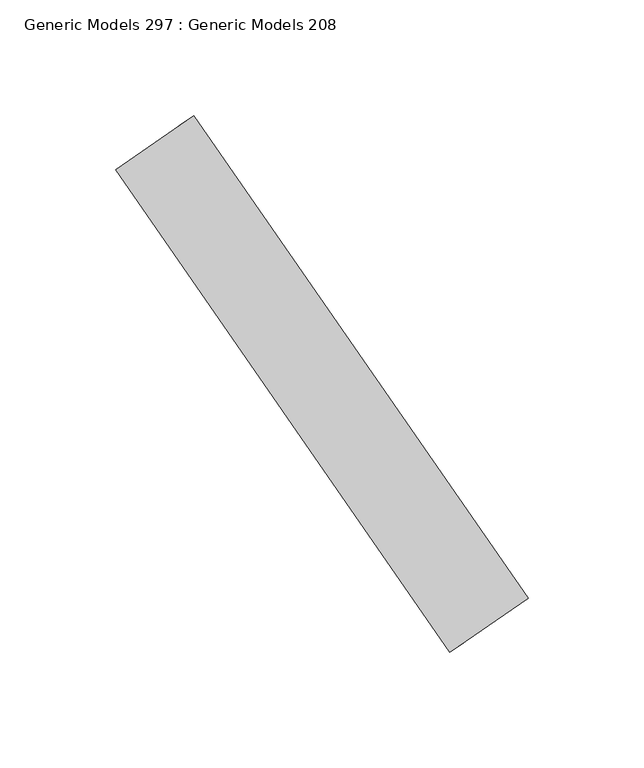
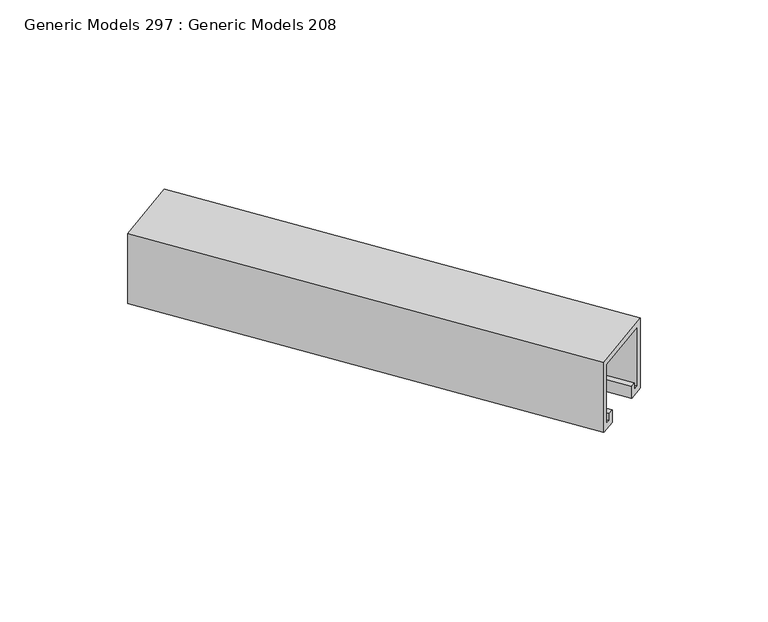
"""IFC4 building model written with IfcOpenShell, lengths in millimetres: proxy geometry, Generic Models 297 : Generic Models 208."""

from ifc_helpers import new_model, si_unit, frame, origin, place, context, project, spatial, polyline, outline, extrude, source, transform, mapped, element, save


def generic_models_297_generic_models_208_0078fd4a(model_context):
    return source(origin(), model_context, "Body", "SweptSolid", [
        extrude(outline(polyline([(-3.175, 0.0), (-3.175, 34.925), (-38.1, 34.925), (-38.1, 31.75), (-34.13125, 31.75), (-34.13125, 28.5750001), (-41.275, 28.5750001), (-41.275, 38.1), (0.0, 38.1), (0.0, -3.175), (-41.275, -3.175), (-41.275, 6.35), (-34.13125, 6.35), (-34.13125, 3.175), (-38.1, 3.175), (-38.1, 0.0), (-3.175, 0.0)])), frame((-2463.8722582, -22814.1902031, 1035.05), z_axis=(-0.5693796736417774, 0.8220746847115432, 0.0), x_axis=(0.0, 0.0, 1.0)), (0.0, 0.0, 1.0), 254.0),
    ])


if __name__ == "__main__":
    model = new_model("IFC4")
    model_context = context("Model", 3, world=origin())
    ifc_project = project(units=[si_unit("LENGTHUNIT", "METRE", prefix="MILLI")], contexts=[model_context])
    site = spatial("IfcSite", under=ifc_project)
    building = spatial("IfcBuilding", under=site)
    placement = place(None, origin())
    generic_models_297_generic_models_208_shape = generic_models_297_generic_models_208_0078fd4a(model_context)
    element("IfcBuildingElementProxy", 1, Name="Generic Models 297 : Generic Models 208", ObjectType="Generic Models 297 : Generic Models 208", at=placement, inside=building, context=model_context, shape_type="MappedRepresentation", body=[
        mapped(generic_models_297_generic_models_208_shape, transform((0.0, 0.0, 0.0), x_axis=(1.0, 0.0, 0.0), y_axis=(0.0, 1.0, 0.0), z_axis=(0.0, 0.0, 1.0))),
    ])
    save(model, "model.ifc")

# Revit data of these elements
# Project information
#   Project Issue Date = "03.10.2017"
#   Project Status = "Project Status"
#   Client Name = "Owner"
#   Project Address = "5964 Executive Dr, Fitchburg, WI 53719"
#   Project Name = "Infinite Athlete"
#   Project Number = "Project Number"
# Element 1 (IfcBuildingElementProxy, "Generic Models 297 : Generic Models 208")
#   Materials on its faces: "UNISTRUT P1000, 1 5/8\" X 1 5/8\", CHANNEL OR ALUM. CHANNEL"
# Materials
#   "UNISTRUT P1000, 1 5/8\" X 1 5/8\", CHANNEL OR ALUM. CHANNEL": class "Metal", colour RGB 244 244 244, transparency 0, Description = "Aluminum 6061", Cost = 0
